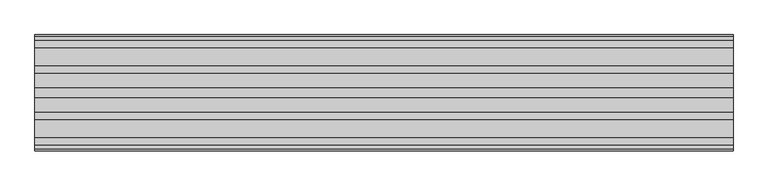
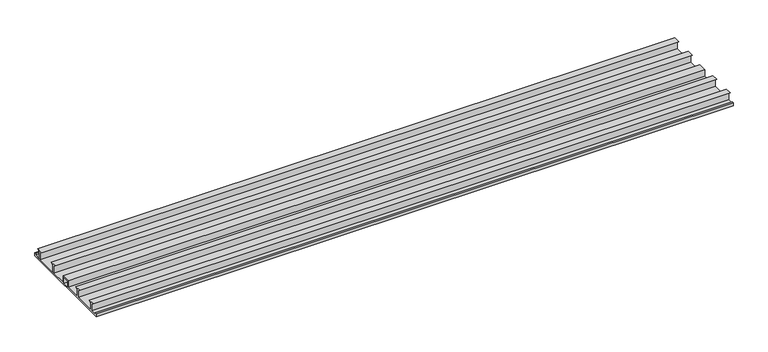
"""IFC4 building model written with IfcOpenShell, lengths in millimetres: proxy geometry, TN_Гидрошпонка ТН Фундамент : Гидрошпонка ТН Фундамент ДШ-Н-250."""

from ifc_helpers import new_model, si_unit, frame, origin, place, context, project, spatial, polyline, outline, extrude, source, transform, mapped, element, save


def specialty_equipment_ac09f71f(model_context):
    return source(origin(), model_context, "Body", "SweptSolid", [
        extrude(outline(polyline([(125.0, 0.0), (-125.0, 0.0), (-125.0, 7.9804873), (-122.0, 7.9804873), (-122.0, 4.0), (-107.0456593, 4.0), (-107.0456593, 22.012356), (-112.5, 25.0), (-97.5, 25.0), (-102.9543407, 22.012356), (-102.9543407, 4.0), (-52.0456593, 4.0), (-52.0456593, 22.012356), (-57.5, 25.0), (-42.5, 25.0), (-47.9543407, 22.012356), (-47.9543407, 4.0), (-10.0, 4.0), (-10.0, 20.0), (10.0, 20.0), (10.0, 4.0), (47.9543407, 4.0), (47.9543407, 22.012356), (42.5, 25.0), (57.5, 25.0), (52.0456593, 22.012356), (52.0456593, 4.0), (102.9543407, 4.0), (102.9543407, 22.012356), (97.5, 25.0), (112.5, 25.0), (107.0456593, 22.012356), (107.0456593, 4.0), (122.0, 4.0), (122.0, 7.9804873), (125.0, 7.9804873), (125.0, 0.0)]), holes=[polyline([(-7.0213922, 17.012356), (-7.0213922, 2.7793951), (7.0213922, 2.7793951), (7.0213922, 17.012356), (-7.0213922, 17.012356)])]), frame((0.0, 0.0, 0.0), z_axis=(1.0, 0.0, 0.0), x_axis=(0.0, 1.0, 0.0)), (0.0, 0.0, 1.0), 1500.0),
    ])


if __name__ == "__main__":
    model = new_model("IFC4")
    model_context = context("Model", 3, world=origin())
    ifc_project = project(units=[si_unit("LENGTHUNIT", "METRE", prefix="MILLI")], contexts=[model_context])
    site = spatial("IfcSite", under=ifc_project)
    building = spatial("IfcBuilding", under=site)
    placement = place(None, origin())
    specialty_equipment_shape = specialty_equipment_ac09f71f(model_context)
    element("IfcBuildingElementProxy", 1, Name="TN_Гидрошпонка ТН Фундамент : Гидрошпонка ТН Фундамент ДШ-Н-250", ObjectType="TN_Гидрошпонка ТН Фундамент : Гидрошпонка ТН Фундамент ДШ-Н-250", at=placement, inside=building, context=model_context, shape_type="MappedRepresentation", body=[
        mapped(specialty_equipment_shape, transform((0.0, 0.0, 0.0), x_axis=(1.0, 0.0, 0.0), y_axis=(0.0, 1.0, 0.0), z_axis=(0.0, 0.0, 1.0))),
    ])
    save(model, "model.ifc")

# Revit data of these elements
# Type "TN_Гидрошпонка ТН Фундамент : Гидрошпонка ТН Фундамент ДШ-Н-250"
#   Description = "Наружные гидроизоляционные шпонки ТН Фундамент ДШ-Н предназначены для герметизации деформационных швов бетонирования при строительстве подземных и заглубленных конструкций зданий и сооружений различного назначения и класса ответственности."
#   Type Comments = "п.м."
#   Manufacturer = "ТехноНИКОЛЬ"
#   URL = "https://nav.tn.ru/catalog/gidroizolyatsiya/komplektatsiya-dlya-gidroizolyatsii/gidroshponki-tekhnonikol-fundament-dsh-n/"
#   ADSK_Примечание = ""
#   ADSK_Обозначение [instance default] = "ТехноНИКОЛЬ"
#   ADSK_Наименование = "Гидрошпонка ТН Фундамент ДШ-Н-250"
#   ADSK_Масса_Текст = ""
#   ADSK_Марка = ""
#   ADSK_Код изделия = "66671"
#   ADSK_Завод-изготовитель [instance default] = "ТехноНИКОЛЬ"
#   ADSK_Единица измерения [instance default] = "п.м."
#   ADSK_Группирование = "Гидрошпонки"
#   ADSK_URL страницы изделия = "https://nav.tn.ru/catalog/gidroizolyatsiya/komplektatsiya-dlya-gidroizolyatsii/gidroshponki-tekhnonikol-fundament-dsh-n/"
#   ADSK_URL документации изделия = "https://nav.tn.ru/upload/iblock/ec5/xbb24x1u8yp3edzrrex0jfnnntpjibsj/Tekhlist-7.399_Gidroshponki-TN-Fundament-DSH_N_RU_ru.pdf"
#   built-in parameter 1001306 [instance default] = 3.28084 (stored number, unit not read)
#   ADSK_Размер_Длина [instance default] = 1000 mm
#   ADSK_Количество [instance default] = 1
#   Гидрошпонка ТН Фундамент ТШ-Н-210 = no
#   Гидрошпонка ТН Фундамент ДШП-В-50 = no
#   Гидрошпонка ТН Фундамент ДШП-В-20 = no
#   Гидрошпонка ТН Фундамент ДШ-В-280 = no
#   Гидрошпонка ТН Фундамент ДШ-В-250 = no
#   Гидрошпонка ТН Фундамент ТШ-В-250 = no
#   Гидрошпонка ТН Фундамент ТПС-В 140-1 = no
#   Гидрошпонка ТН Фундамент ДШ-Н-280 = no
#   Гидрошпонка ТН Фундамент ДШ-Н-250 = yes
#   Гидрошпонка ТН Фундамент ТПС-В 100-2 = no
#   Гидрошпонка ТН Фундамент ТШ-Н-250 = no
#   Гидрошпонка ТН Фундамент ТШ-В-210 = no
#   Материал = TN_ПВХ_Черный
#   Default Elevation = 0
# Element 1 (IfcBuildingElementProxy, "TN_Гидрошпонка ТН Фундамент : Гидрошпонка ТН Фундамент ДШ-Н-250")
#   built-in parameter 1001306 = 4.92126 (stored number, unit not read)
#   ADSK_Размер_Длина = 1500 mm
#   ADSK_Количество = 1.5
#   Materials on its faces: "TN_ПВХ_Черный"
# Materials
#   "TN_ПВХ_Черный": class "Типовые", colour RGB 48 48 48, transparency 0, Cost = 0
